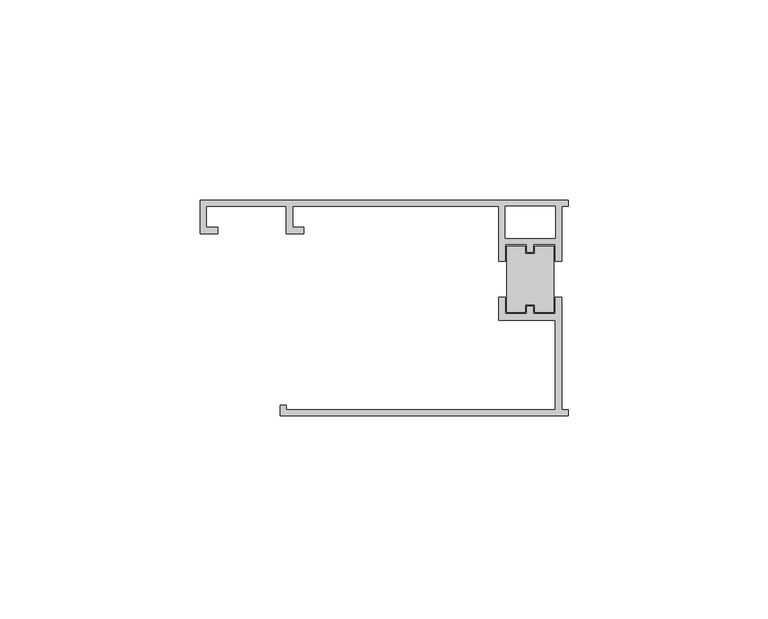
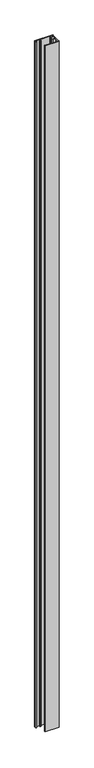
"""IFC4 building model written with IfcOpenShell, lengths in millimetres: proxy geometry, Generic Models 2:Generic Models 2:310765:Generic Models 2:310765 : Generic Models 2:Generic Models 2:310765:9 : Generic Models 2:Generic Models 2:310765:Generic Models 2:310765 : Generic Models 2:Generic Models 2:310765:300385."""

from ifc_helpers import new_model, si_unit, frame, origin, place, context, project, spatial, polyline, outline, extrude, source, transform, mapped, element, save


def generic_models_73402b5a(model_context):
    return source(origin(), model_context, "Body", "SweptSolid", [
        extrude(outline(polyline([(564983.3960122, -568246.416762), (564983.3960122, -568229.8645058), (564988.0935108, -568229.8645058), (564988.0935108, -568231.7899212), (564990.4747608, -568231.7899212), (564990.4747608, -568229.8645058), (564995.1722595, -568229.8645058), (564995.1722595, -568246.416762), (564990.4747608, -568246.416762), (564990.4747608, -568244.4913465), (564988.0935108, -568244.4913465), (564988.0935108, -568246.416762), (564983.3960122, -568246.416762)])), frame((0.0, 0.0, 4892.1011248), z_axis=(0.0, 0.0, 1.0), x_axis=(1.0, 0.0, 0.0)), (0.0, 0.0, 1.0), 3663.6668744),
        extrude(outline(polyline([(564906.7441345, -568226.7958673), (564906.7441345, -568218.3494958), (564998.7441345, -568218.3494958), (564998.7441345, -568219.9369958), (564997.1566345, -568219.9369958), (564997.1566345, -568233.6348183), (564995.5691345, -568233.6348183), (564995.5691345, -568229.4676308), (564990.0778858, -568229.4676308), (564990.0778858, -568231.3930462), (564988.4903858, -568231.3930462), (564988.4903858, -568229.4676308), (564982.9991372, -568229.4676308), (564982.9991372, -568233.6348183), (564981.4116372, -568233.6348183), (564981.4116372, -568219.9369958), (564929.9191345, -568219.9369958), (564929.9191345, -568225.2083673), (564932.718961, -568225.2083673), (564932.718961, -568226.7958673), (564928.3316345, -568226.7958673), (564928.3316345, -568219.9369958), (564908.3316345, -568219.9369958), (564908.3316345, -568225.2083673), (564911.131461, -568225.2083673), (564911.131461, -568226.7958673), (564906.7441345, -568226.7958673)]), holes=[polyline([(564982.9991372, -568219.9369958), (564982.9991372, -568227.8801308), (564995.5691345, -568227.8801308), (564995.5691345, -568219.9369958), (564982.9991372, -568219.9369958)])]), frame((0.0, 0.0, 4892.1011248), z_axis=(0.0, 0.0, 1.0), x_axis=(1.0, 0.0, 0.0)), (0.0, 0.0, 1.0), 3663.6668744),
        extrude(outline(polyline([(564998.7441345, -568270.7619958), (564998.7441345, -568272.3494958), (564926.7441345, -568272.3494958), (564926.7441345, -568269.6344059), (564928.3316345, -568269.6344059), (564928.3316345, -568270.7619958), (564995.5691345, -568270.7619958), (564995.5691345, -568248.401137), (564981.4116372, -568248.401137), (564981.4116372, -568242.6464495), (564982.9991372, -568242.6464495), (564982.9991372, -568246.813637), (564988.4903858, -568246.813637), (564988.4903858, -568244.8882215), (564990.0778858, -568244.8882215), (564990.0778858, -568246.813637), (564995.5691345, -568246.813637), (564995.5691345, -568242.6464495), (564997.1566345, -568242.6464495), (564997.1566345, -568270.7619958), (564998.7441345, -568270.7619958)])), frame((0.0, 0.0, 4892.1011248), z_axis=(0.0, 0.0, 1.0), x_axis=(1.0, 0.0, 0.0)), (0.0, 0.0, 1.0), 3663.6668744),
    ])


if __name__ == "__main__":
    model = new_model("IFC4")
    model_context = context("Model", 3, world=origin())
    ifc_project = project(units=[si_unit("LENGTHUNIT", "METRE", prefix="MILLI")], contexts=[model_context])
    site = spatial("IfcSite", under=ifc_project)
    building = spatial("IfcBuilding", under=site)
    placement = place(None, origin())
    generic_models_shape = generic_models_73402b5a(model_context)
    element("IfcBuildingElementProxy", 1, Name="Generic Models 2:Generic Models 2:310765:Generic Models 2:310765 : Generic Models 2:Generic Models 2:310765:9 : Generic Models 2:Generic Models 2:310765:Generic Models 2:310765 : Generic Models 2:Generic Models 2:310765:300385", ObjectType="Generic Models 2:Generic Models 2:310765:Generic Models 2:310765 : Generic Models 2:Generic Models 2:310765:9 : Generic Models 2:Generic Models 2:310765:Generic Models 2:310765 : Generic Models 2:Generic Models 2:310765:300385", at=placement, inside=building, context=model_context, shape_type="MappedRepresentation", body=[
        mapped(generic_models_shape, transform((0.0, 0.0, 0.0), x_axis=(1.0, 0.0, 0.0), y_axis=(0.0, 1.0, 0.0), z_axis=(0.0, 0.0, 1.0))),
    ])
    save(model, "model.ifc")

# Revit data of these elements
# Type "Generic Models 2:Generic Models 2:310765:Generic Models 2:310765 : Generic Models 2:Generic Models 2:310765:9 : Generic Models 2:Generic Models 2:310765:Generic Models 2:310765 : Generic Models 2:Generic Models 2:310765:300385"
#   NameOverride = "Generic Models 2:Generic Models 2:310765:Generic Models 2:310765 : Generic Models 2:Generic Models 2:310765:300385"
#   ObjectTypeOverride = "Generic Models 2:310765 : Generic Models 2:Generic Models 2:310765"
#   Reference = "Generic Models 2"
#   Tag = "300385"
# Element 1 (IfcBuildingElementProxy, "Generic Models 2:Generic Models 2:310765:Generic Models 2:310765 : Generic Models 2:Generic Models 2:310765:9 : Generic Models 2:Generic Models 2:310765:Generic Models 2:310765 : Generic Models 2:Generic Models 2:310765:300385")
#   Materials on its faces: "THERMAL BROKEN ALUMINUM STOREFRONT FOR POLYCARBONATE"
# Materials
#   "THERMAL BROKEN ALUMINUM STOREFRONT FOR POLYCARBONATE": class "Unassigned", colour RGB 244 244 244, transparency 0, Keynote = "M07611300.01", Cost = 0
